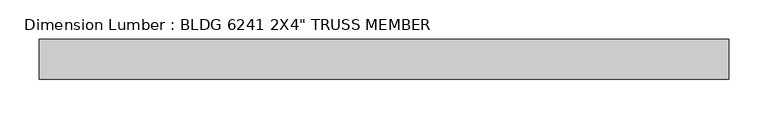
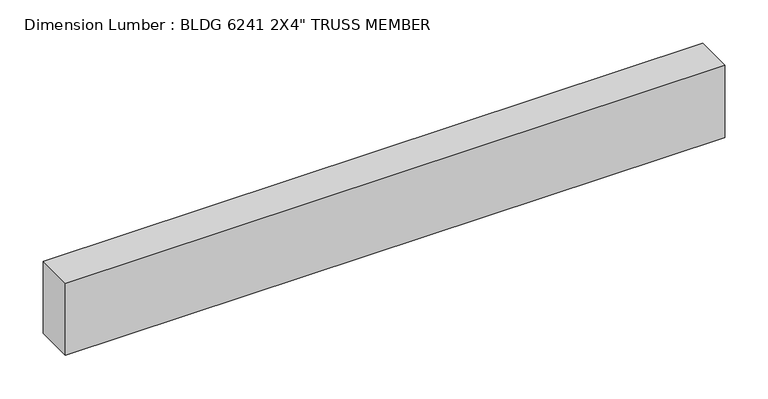
"""IFC4 building model written with IfcOpenShell, lengths in millimetres: beam geometry."""

from ifc_helpers import new_model, si_unit, frame, origin, place, context, project, spatial, polyline, outline, extrude, source, transform, mapped, element, save


def beam_e0e1cdb9(model_context):
    return source(origin(), model_context, "Body", "SweptSolid", [
        extrude(outline(polyline([(444.5, 25.4), (444.5, -25.4), (-431.7999994, -25.4), (-431.7999994, 25.4), (444.5, 25.4)])), frame((0.0, 0.0, -50.8), z_axis=(0.0, 0.0, 1.0), x_axis=(1.0, 0.0, 0.0)), (0.0, 0.0, 1.0), 101.6),
    ])


if __name__ == "__main__":
    model = new_model("IFC4")
    model_context = context("Model", 3, world=origin())
    ifc_project = project(units=[si_unit("LENGTHUNIT", "METRE", prefix="MILLI")], contexts=[model_context])
    site = spatial("IfcSite", under=ifc_project)
    building = spatial("IfcBuilding", under=site)
    placement = place(None, origin())
    beam_shape = beam_e0e1cdb9(model_context)
    element("IfcBeam", 1, ObjectType="Dimension Lumber : BLDG 6241 2X4\" TRUSS MEMBER", at=placement, inside=building, context=model_context, shape_type="MappedRepresentation", body=[
        mapped(beam_shape, transform((0.0, 0.0, 0.0), x_axis=(1.0, 0.0, 0.0), y_axis=(0.0, 1.0, 0.0), z_axis=(0.0, 0.0, 1.0))),
    ])
    save(model, "model.ifc")

# Revit data of these elements
# Type "Dimension Lumber : BLDG 6241 2X4\" TRUSS MEMBER"
#   Assembly Code = "B10"
#   A = 0.273472 SF
#   Length [instance default] = 5' - 0"
#   b = 0' - 2"
#   d = 0' - 4"
#   Structural Material [instance default] = Softwood, Lumber
# Element 1 (IfcBeam, "Dimension Lumber : BLDG 6241 2X4\" TRUSS MEMBER")
#   Materials on its faces: "Softwood, Lumber"
# Materials
#   "Softwood, Lumber": class "Wood", colour RGB 223 192 134, transparency 0, Description = "Pinus Echinata", Cost = 0
